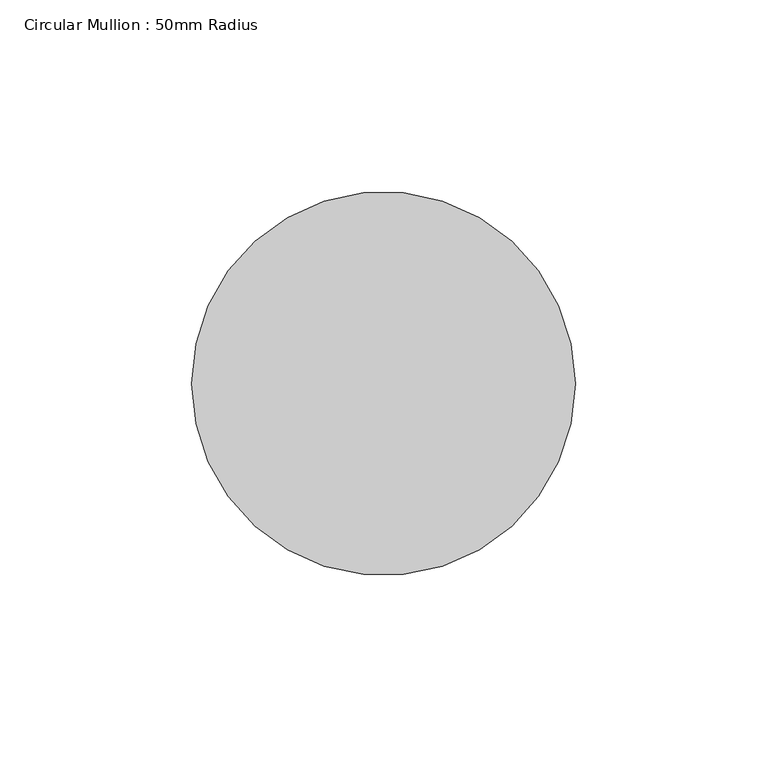
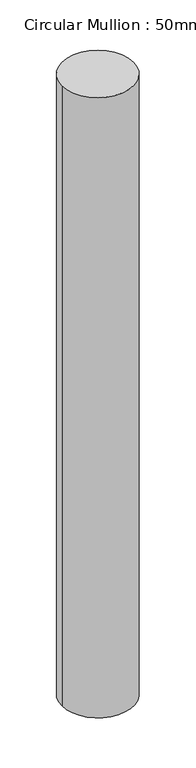
"""IFC4 building model written with IfcOpenShell, lengths in millimetres: member geometry, Circular Mullion : 50mm Radius."""

from ifc_helpers import new_model, si_unit, point, frame, origin, origin_2d, place, context, project, spatial, circle_curve, trimmed, segment, composite_curve, outline, extrude, source, transform, mapped, element, save


def circular_mullion_50mm_radius_e2d26305(model_context):
    return source(origin(), model_context, "Body", "SweptSolid", [
        extrude(outline(composite_curve([segment(trimmed(circle_curve(origin_2d(), 50.0), [point((50.0, 0.0))], [point((-50.0, 0.0))], False, "CARTESIAN"), True, "CONTINUOUS"), segment(trimmed(circle_curve(origin_2d(), 50.0), [point((-50.0, 0.0))], [point((50.0, 0.0))], False, "CARTESIAN"), True, "CONTINUOUS")], self_intersect=False)), frame((0.0, 0.0, -913.5515333), z_axis=(0.0, 0.0, 1.0), x_axis=(1.0, 0.0, 0.0)), (0.0, 0.0, 1.0), 913.5515333),
    ])


if __name__ == "__main__":
    model = new_model("IFC4")
    model_context = context("Model", 3, world=origin())
    ifc_project = project(units=[si_unit("LENGTHUNIT", "METRE", prefix="MILLI")], contexts=[model_context])
    site = spatial("IfcSite", under=ifc_project)
    building = spatial("IfcBuilding", under=site)
    placement = place(None, origin())
    circular_mullion_50mm_radius_shape = circular_mullion_50mm_radius_e2d26305(model_context)
    element("IfcMember", 1, ObjectType="Circular Mullion : 50mm Radius", at=placement, inside=building, context=model_context, shape_type="MappedRepresentation", body=[
        mapped(circular_mullion_50mm_radius_shape, transform((0.0, 0.0, 0.0), x_axis=(1.0, 0.0, 0.0), y_axis=(0.0, 1.0, 0.0), z_axis=(0.0, 0.0, 1.0))),
    ])
    save(model, "model.ifc")

# Revit data of these elements
# Type "Circular Mullion : 50mm Radius"
#   built-in parameter 1007350 = 0.164042 (stored number, unit not read)
# Element 1 (IfcMember, "Circular Mullion : 50mm Radius")
#   Materials on its faces: "Aluminium"
# Materials
#   "Aluminium": class "Metal", colour RGB 247 247 247, transparency 0, Description = "Aluminium 6061", Cost = 0
